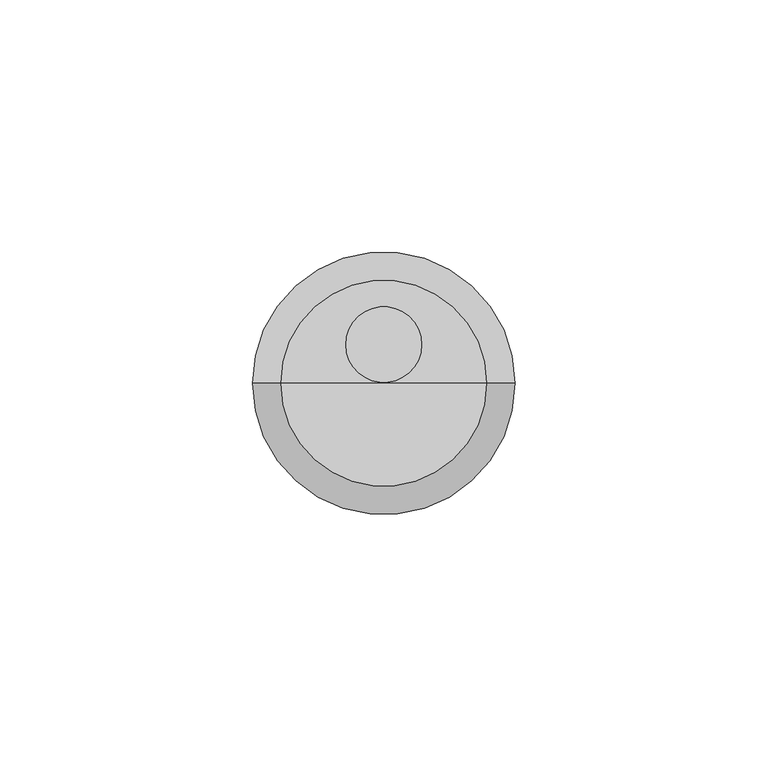
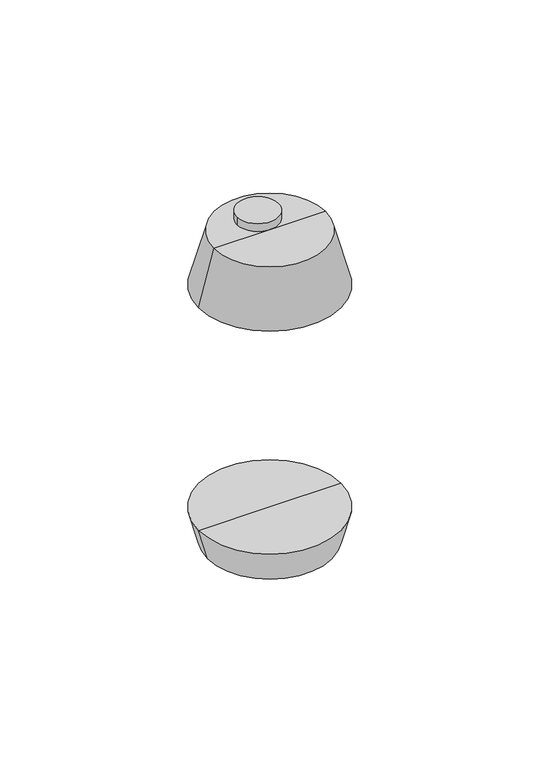
"""IFC4 building model written with IfcOpenShell, lengths in millimetres: proxy geometry, Architectural Hardware_1745 Triton_ASSA ABLOY_9217043AB01A02 : 1745 Triton_9217043AB01A02."""

from ifc_helpers import new_model, si_unit, point, frame, frame_2d, origin, place, context, project, spatial, polyline, circle_curve, trimmed, segment, composite_curve, outline, extrude, source, transform, mapped, element, save
from ifc_brep_helpers import plane_surface, revolved_surface, advanced_brep


def specialty_equipment_88dc195d(model_context):
    return source(origin(), model_context, "Body", "SolidModel", [
        extrude(outline(composite_curve([segment(trimmed(circle_curve(frame_2d((0.0, 7.6487032)), 7.5), [point((0.0, 0.1487032))], [point((0.0, 15.1487032))], False, "CARTESIAN"), True, "CONTINUOUS"), segment(trimmed(circle_curve(frame_2d((0.0, 7.6487032)), 7.5), [point((0.0, 15.1487032))], [point((0.0, 0.1487032))], False, "CARTESIAN"), True, "CONTINUOUS")], self_intersect=False)), frame((0.0, 0.0, -101.0), z_axis=(0.0, 0.0, 1.0), x_axis=(1.0, 0.0, 0.0)), (0.0, 0.0, 1.0), 3.0),
        advanced_brep(
        [(22.7698592, 0.0, -98.0), (25.9852495, 0.0, -86.0), (-25.9852495, 0.0, -86.0), (-22.7698592, 0.0, -98.0), (0.0, 0.0, -98.0), (0.0, 0.0, -86.0)],
        [
            (0, 1),
            (1, 2, circle_curve(frame((0.0, 0.0, -86.0), z_axis=(0.0, 0.0, -1.0), x_axis=(-1.0, 0.0, 0.0)), 25.9852495)),
            (2, 3),
            (3, 0, circle_curve(frame((0.0, 0.0, -98.0), z_axis=(0.0, 0.0, 1.0), x_axis=(-1.0, 0.0, 0.0)), 22.7698592)),
            (2, 1, circle_curve(frame((0.0, 0.0, -86.0), z_axis=(0.0, 0.0, -1.0), x_axis=(-1.0, 0.0, 0.0)), 25.9852495)),
            (0, 3, circle_curve(frame((0.0, 0.0, -98.0), z_axis=(0.0, 0.0, 1.0), x_axis=(-1.0, 0.0, 0.0)), 22.7698592)),
            (4, 0),
            (3, 4),
            (1, 5),
            (5, 2),
        ],
        [
            revolved_surface(polyline([(-25.9852495, 0.0, -86.0), (-22.7698592, 0.0, -98.0)]), (0.0, 0.0, -111.4021567), (0.0, 0.0, -1.0)),
            plane_surface(frame((0.0, 0.0, -98.0), z_axis=(0.0, 0.0, -1.0), x_axis=(-1.0, 0.0, 0.0))),
            plane_surface(frame((0.0, 0.0, -86.0), z_axis=(0.0, 0.0, 1.0), x_axis=(-1.0, 0.0, 0.0))),
        ],
        [
            (0, [[1, 2, 3, 4]]),
            (0, [[-3, 5, -1, 6]]),
            (1, [[7, -4, 8]]),
            (1, [[-8, -6, -7]]),
            (2, [[9, 10, -2]]),
            (2, [[-10, -9, -5]]),
        ],
    ),
        extrude(outline(composite_curve([segment(trimmed(circle_curve(frame_2d((0.0, 7.6487032)), 7.5), [point((-7.5, 7.6487032))], [point((7.5, 7.6487032))], False, "CARTESIAN"), True, "CONTINUOUS"), segment(trimmed(circle_curve(frame_2d((0.0, 7.6487032)), 7.5), [point((7.5, 7.6487032))], [point((-7.5, 7.6487032))], False, "CARTESIAN"), True, "CONTINUOUS")], self_intersect=False)), frame((0.0, 0.0, 21.0), z_axis=(0.0, 0.0, 1.0), x_axis=(1.0, 0.0, 0.0)), (0.0, 0.0, 1.0), 3.0),
        advanced_brep(
        [(0.0, 0.0, 0.0), (26.0, 0.0, 0.0), (-26.0, 0.0, 0.0), (20.373067, 0.0, 21.0), (0.0, 0.0, 21.0), (-20.373067, 0.0, 21.0)],
        [
            (0, 1),
            (1, 2, circle_curve(frame((0.0, 0.0, 0.0), z_axis=(0.0, 0.0, -1.0), x_axis=(-1.0, 0.0, 0.0)), 26.0)),
            (2, 0),
            (2, 1, circle_curve(frame((0.0, 0.0, 0.0), z_axis=(0.0, 0.0, -1.0), x_axis=(-1.0, 0.0, 0.0)), 26.0)),
            (3, 4),
            (4, 5),
            (5, 3, circle_curve(frame((0.0, 0.0, 21.0), z_axis=(0.0, 0.0, 1.0), x_axis=(-1.0, 0.0, 0.0)), 20.373067)),
            (3, 5, circle_curve(frame((0.0, 0.0, 21.0), z_axis=(0.0, 0.0, 1.0), x_axis=(-1.0, 0.0, 0.0)), 20.373067)),
            (1, 3),
            (5, 2),
        ],
        [
            plane_surface(frame((0.0, 0.0, 0.0), z_axis=(0.0, 0.0, -1.0), x_axis=(-1.0, 0.0, 0.0))),
            plane_surface(frame((0.0, 0.0, 21.0), z_axis=(0.0, 0.0, 1.0), x_axis=(-1.0, 0.0, 0.0))),
            revolved_surface(polyline([(-20.373067, 0.0, 21.0), (-26.0, 0.0, 0.0)]), (0.0, 0.0, 55.0698043), (0.0, 0.0, -1.0)),
        ],
        [
            (0, [[1, 2, 3]]),
            (0, [[-3, 4, -1]]),
            (1, [[5, 6, 7]]),
            (1, [[-6, -5, 8]]),
            (2, [[9, -7, 10, -2]]),
            (2, [[-10, -8, -9, -4]]),
        ],
    ),
    ])


if __name__ == "__main__":
    model = new_model("IFC4")
    model_context = context("Model", 3, world=origin())
    ifc_project = project(units=[si_unit("LENGTHUNIT", "METRE", prefix="MILLI")], contexts=[model_context])
    site = spatial("IfcSite", under=ifc_project)
    building = spatial("IfcBuilding", under=site)
    placement = place(None, origin())
    specialty_equipment_shape = specialty_equipment_88dc195d(model_context)
    element("IfcBuildingElementProxy", 1, Name="Architectural Hardware_1745 Triton_ASSA ABLOY_9217043AB01A02 : 1745 Triton_9217043AB01A02", ObjectType="Architectural Hardware_1745 Triton_ASSA ABLOY_9217043AB01A02 : 1745 Triton_9217043AB01A02", at=placement, inside=building, context=model_context, shape_type="MappedRepresentation", body=[
        mapped(specialty_equipment_shape, transform((0.0, 0.0, 0.0), x_axis=(1.0, 0.0, 0.0), y_axis=(0.0, 1.0, 0.0), z_axis=(0.0, 0.0, 1.0))),
    ])
    save(model, "model.ifc")

# Revit data of these elements
# Type "Architectural Hardware_1745 Triton_ASSA ABLOY_9217043AB01A02 : 1745 Triton_9217043AB01A02"
#   Uniclass 2.0 Description = "Door Locks"
#   Uniclass 2.0 Code = "PR-36-08-22"
#   Uniclass 1.4 Description = "Door furniture"
#   Uniclass 1.4 Code = "L4181"
#   URL = "http://assaabloyopeningsolutions.no/prosjekt"
#   UNSPSC Code = ""
#   Type Comments = "1745 Triton"
#   Region Europe = "NO"
#   Reference Standards = "NS-EN 1303"
#   Provider = " ASSA ABLOY Opening Solutions Norway\r\n"
#   Product Range = "Triton"
#   Product Guid = "e7b73694-14dc-46e7-844e-fe8781a7c773"
#   Product Group = "Cylinders"
#   Product Datasheet = "http://xnet.trioving.be/Katalog.asp?ProdId=199996"
#   OmniClass Description = "Door Latches"
#   OmniClass Code = "23-17 19 11 21 19"
#   Name = "1745 Triton"
#   NBS Reference Description = "Door Locks"
#   NBS Reference Code = "36-08-22"
#   Model = "Architectural Hardware_1745 Triton_ASSA ABLOY_9217043AB01A02"
#   Manufacturer = "ASSA ABLOY"
#   ISO = "ISO 14001"
#   IFC Classification = ""
#   Environmental Product Declaration (EPD) = ""
#   Description = "Cylinder Set Oval  w/ Round Escutcheon and w/ Turn on One Side"
#   Date of publishing = "2015-11-16"
#   Contact Provider = "http://assaabloyopeningsolutions.no/prosjekt"
#   BIMobject category = "Door Hardware"
#   BIMobject Unique ref = "9217043AB01A02"
#   BIMobject Instructions Video = "https://www.youtube.com/user/BIMobject"
#   BIMobject Brand = "ASSA ABLOY NO"
#   Article Number = "9217043AB01A02"
#   Accessories = ""
#   Offset = 0' - 1.9685"
#   Door Panel Thickness [instance default] = 0' - 1.5748"
#   Thumb Turn = no
#   Edition number = 2
#   Cylinder = yes
#   1745 Triton [instance default] = no
#   Finish = Satin Chrome
#   Default Elevation = 0
#   Cost = 0
# Element 1 (IfcBuildingElementProxy, "Architectural Hardware_1745 Triton_ASSA ABLOY_9217043AB01A02 : 1745 Triton_9217043AB01A02")
#   Door Panel Thickness = 0' - 3.38583"
#   Materials on its faces: "Satin Chrome"
# Materials
#   "Satin Chrome": class "Metal", colour RGB 244 244 244, transparency 0, Description = "Satin Chrome", Cost = 0
